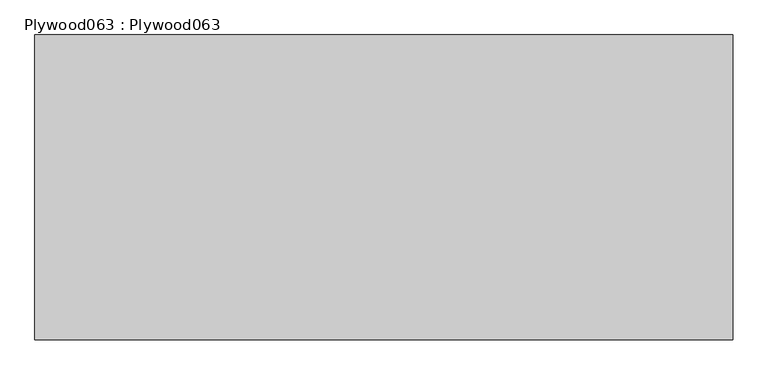
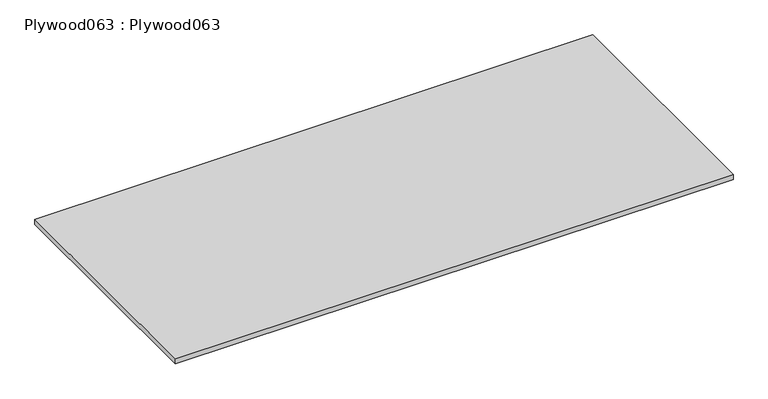
"""IFC4 building model written with IfcOpenShell, lengths in millimetres: proxy geometry, Plywood063 : Plywood063."""

import ifcopenshell
import ifcopenshell.guid

model = None  # the IFC model being written
_history = None  # IfcOwnerHistory: only IFC2X3 demands one
_inside = {}  # id of a spatial element -> (the spatial element, [elements in it])
_under = {}  # id of a project, library or spatial element -> (it, [spatial elements below it])
_declared = {}  # id of a project -> (the project, [libraries it declares])
_typed = {}  # id of a type object -> (the type object, [elements of that type])
_made_of = {}  # id of a material, layer set ... -> (it, [elements and type objects made of it])


def new_model(schema):
    """Start an empty IFC model of exactly this schema.

    Asked for "IFC4X3", IfcOpenShell would pick the latest addendum, in which some entities
    have other attributes; the version numbers below select the first issue.
    IFC2X3 requires an IfcOwnerHistory on every rooted entity: one is made here for all.
    """
    global model, _history
    if schema == "IFC4X3":
        model = ifcopenshell.file(schema_version=(4, 3, 0, 0))
    else:
        model = ifcopenshell.file(schema=schema)
    _inside.clear()
    _under.clear()
    _declared.clear()
    _typed.clear()
    _made_of.clear()
    _history = None
    if model.schema == "IFC2X3":
        org = make("IfcOrganization", Name="unknown")
        user = make(
            "IfcPersonAndOrganization",
            ThePerson=make("IfcPerson", FamilyName="unknown"),
            TheOrganization=org,
        )
        app = make(
            "IfcApplication",
            ApplicationDeveloper=org,
            Version="unknown",
            ApplicationFullName="unknown",
            ApplicationIdentifier="unknown",
        )
        _history = make(
            "IfcOwnerHistory",
            OwningUser=user,
            OwningApplication=app,
            ChangeAction="ADDED",
            CreationDate=0,
        )
    return model


def make(cls, **values):
    """One entity of the class cls with the attributes given. An attribute that is None is left unset."""
    return model.create_entity(
        cls, **{name: value for name, value in values.items() if value is not None}
    )


def rooted(cls, **values):
    """An entity with a GlobalId (a new one), such as an element, a storey or a relation."""
    return make(cls, GlobalId=ifcopenshell.guid.new(), OwnerHistory=_history, **values)


def si_unit(unit_type, name, prefix=None):
    """IfcSIUnit, for example si_unit("LENGTHUNIT", "METRE", prefix="MILLI")."""
    return make("IfcSIUnit", UnitType=unit_type, Prefix=prefix, Name=name)


def assignment(units):
    """IfcUnitAssignment: the units of a project."""
    return None if units is None else make("IfcUnitAssignment", Units=units)


def point(xyz):
    """IfcCartesianPoint."""
    return None if xyz is None else make("IfcCartesianPoint", Coordinates=xyz)


def direction(xyz):
    """IfcDirection."""
    return None if xyz is None else make("IfcDirection", DirectionRatios=xyz)


def frame(location, z_axis=None, x_axis=None):
    """IfcAxis2Placement3D, a coordinate frame: its origin and axes. An axis left out is left unset."""
    return make(
        "IfcAxis2Placement3D",
        Location=point(location),
        Axis=direction(z_axis),
        RefDirection=direction(x_axis),
    )


def origin():
    """The frame at (0, 0, 0) with its axes left unset."""
    return frame((0.0, 0.0, 0.0))


def place(relative_to, where):
    """IfcLocalPlacement: puts the frame where relative to a parent placement (None: the world)."""
    return make(
        "IfcLocalPlacement", PlacementRelTo=relative_to, RelativePlacement=where
    )


def context(
    kind, dimensions, precision=None, world=None, true_north=None, identifier=None
):
    """IfcGeometricRepresentationContext, for example the 3D "Model" context."""
    return make(
        "IfcGeometricRepresentationContext",
        ContextIdentifier=identifier,
        ContextType=kind,
        CoordinateSpaceDimension=dimensions,
        Precision=precision,
        WorldCoordinateSystem=world,
        TrueNorth=true_north,
    )


def project(units=None, contexts=None):
    """IfcProject with its units and contexts."""
    return rooted(
        "IfcProject",
        Name="project",
        RepresentationContexts=contexts,
        UnitsInContext=assignment(units),
    )


def spatial(cls, under=None, at=None, **own):
    """A site, building, storey or space (cls), placed at a placement, below another one or the project."""
    s = rooted(cls, ObjectPlacement=at, **own)
    if under is not None:
        _under.setdefault(under.id(), (under, []))[1].append(s)
    return s


def polyline(points):
    """IfcPolyline through the points."""
    return make("IfcPolyline", Points=[point(p) for p in points])


def outline(outer, holes=None, kind="AREA"):
    """IfcArbitraryClosedProfileDef: a profile drawn as a closed curve; with holes, ...WithVoids."""
    if holes is None:
        return make("IfcArbitraryClosedProfileDef", ProfileType=kind, OuterCurve=outer)
    return make(
        "IfcArbitraryProfileDefWithVoids",
        ProfileType=kind,
        OuterCurve=outer,
        InnerCurves=holes,
    )


def extrude(swept, where, along, depth):
    """IfcExtrudedAreaSolid: the profile swept, set in the frame where, extruded along a direction by depth."""
    return make(
        "IfcExtrudedAreaSolid",
        SweptArea=swept,
        Position=where,
        ExtrudedDirection=direction(along),
        Depth=depth,
    )


def shape(context_of_items, identifier, shape_type, items):
    """IfcShapeRepresentation: the items that make up one representation, for example the "Body"."""
    return make(
        "IfcShapeRepresentation",
        ContextOfItems=context_of_items,
        RepresentationIdentifier=identifier,
        RepresentationType=shape_type,
        Items=items,
    )


def source(mapping_origin, context_of_items, identifier, shape_type, items):
    """IfcRepresentationMap: a shape defined once, which mapped items show again and again."""
    return make(
        "IfcRepresentationMap",
        MappingOrigin=mapping_origin,
        MappedRepresentation=shape(context_of_items, identifier, shape_type, items),
    )


def transform(
    local_origin,
    x_axis=None,
    y_axis=None,
    z_axis=None,
    scale=None,
    scale2=None,
    scale3=None,
    uniform=True,
):
    """IfcCartesianTransformationOperator3D, or its non-uniform kind. x_axis, y_axis, z_axis: its Axis1, 2, 3."""
    if uniform:
        return make(
            "IfcCartesianTransformationOperator3D",
            Axis1=direction(x_axis),
            Axis2=direction(y_axis),
            LocalOrigin=point(local_origin),
            Scale=scale,
            Axis3=direction(z_axis),
        )
    return make(
        "IfcCartesianTransformationOperator3DnonUniform",
        Axis1=direction(x_axis),
        Axis2=direction(y_axis),
        LocalOrigin=point(local_origin),
        Scale=scale,
        Axis3=direction(z_axis),
        Scale2=scale2,
        Scale3=scale3,
    )


def mapped(mapping_source, mapping_target):
    """IfcMappedItem: shows the shape of a source again, moved by a transform."""
    return make(
        "IfcMappedItem", MappingSource=mapping_source, MappingTarget=mapping_target
    )


def made_of(thing, what):
    """Note that an element or type object is made of a material, layer set ...; save() writes the relation."""
    if what is not None:
        _made_of.setdefault(what.id(), (what, []))[1].append(thing)
    return thing


def element(
    cls,
    number,
    at=None,
    inside=None,
    cuts=None,
    type_object=None,
    material=None,
    context=None,
    identifier="Body",
    shape_type=None,
    held_by="IfcProductDefinitionShape",
    body=None,
    shapes=None,
    **own,
):
    """One element of the class cls, such as IfcWall. Its Tag is "e" and its number.

    at: its placement. inside: the storey or other place that contains it. cuts: it is an
    opening in that element (IfcRelVoidsElement). A single representation is given by context,
    identifier, shape_type and body (its items); several are given by shapes. held_by: the class
    of the entity that holds the representations. save() writes the other relations.
    """
    e = rooted(cls, Tag="e%d" % number, ObjectPlacement=at, **own)
    if body is not None:
        shapes = [shape(context, identifier, shape_type, body)]
    if shapes is not None:
        e.Representation = make(held_by, Representations=shapes)
    if inside is not None:
        _inside.setdefault(inside.id(), (inside, []))[1].append(e)
    if cuts is not None:
        rooted(
            "IfcRelVoidsElement", RelatingBuildingElement=cuts, RelatedOpeningElement=e
        )
    if type_object is not None:
        _typed.setdefault(type_object.id(), (type_object, []))[1].append(e)
    return made_of(e, material)


def aggregate(whole, parts):
    """IfcRelAggregates: a whole, such as a stair, and the parts it consists of."""
    return rooted("IfcRelAggregates", RelatingObject=whole, RelatedObjects=parts)


def save(model, path):
    """Write the relations noted so far, then the file.

    IfcRelAggregates (storeys below a building ...), IfcRelContainedInSpatialStructure (elements
    in a storey), IfcRelDefinesByType, IfcRelAssociatesMaterial and IfcRelDeclares: one each for
    every whole, place, type object, material and project.
    """
    for whole, parts in _under.values():
        aggregate(whole, parts)
    for where, things in _inside.values():
        rooted(
            "IfcRelContainedInSpatialStructure",
            RelatedElements=things,
            RelatingStructure=where,
        )
    for kind, things in _typed.values():
        rooted("IfcRelDefinesByType", RelatedObjects=things, RelatingType=kind)
    for what, things in _made_of.values():
        rooted("IfcRelAssociatesMaterial", RelatedObjects=things, RelatingMaterial=what)
    for by, libraries in _declared.values():
        rooted("IfcRelDeclares", RelatingContext=by, RelatedDefinitions=libraries)
    model.write(path)


def plywood063_plywood063_23951365(model_context):
    return source(origin(), model_context, "Body", "SweptSolid", [
        extrude(outline(polyline([(14382.7678845, -4670.4213867), (14382.7678845, -5543.3480267), (12382.7678845, -5543.3480267), (12382.7678845, -4670.4213867), (14382.7678845, -4670.4213867)])), frame((0.0, 0.0, 39728.9941181), z_axis=(0.0, 0.0, 1.0), x_axis=(1.0, 0.0, 0.0)), (0.0, 0.0, 1.0), 19.0511007),
    ])


if __name__ == "__main__":
    model = new_model("IFC4")
    model_context = context("Model", 3, world=origin())
    ifc_project = project(units=[si_unit("LENGTHUNIT", "METRE", prefix="MILLI")], contexts=[model_context])
    site = spatial("IfcSite", under=ifc_project)
    building = spatial("IfcBuilding", under=site)
    placement = place(None, origin())
    plywood063_plywood063_shape = plywood063_plywood063_23951365(model_context)
    element("IfcBuildingElementProxy", 1, Name="Plywood063 : Plywood063", ObjectType="Plywood063 : Plywood063", at=placement, inside=building, context=model_context, shape_type="MappedRepresentation", body=[
        mapped(plywood063_plywood063_shape, transform((0.0, 0.0, 0.0), x_axis=(1.0, 0.0, 0.0), y_axis=(0.0, 1.0, 0.0), z_axis=(0.0, 0.0, 1.0))),
    ])
    save(model, "model.ifc")

# Revit data of these elements
# Type "Plywood063 : Plywood063"
#   NameOverride = "Plywood063"
# Element 1 (IfcBuildingElementProxy, "Plywood063 : Plywood063")
#   Materials on its faces: "CDX PLYWOOD -  SEE STRUCTURAL DWGS"
# Materials
#   "CDX PLYWOOD -  SEE STRUCTURAL DWGS": class "Unassigned", colour RGB 177 130 114, transparency 0, Cost = 0
